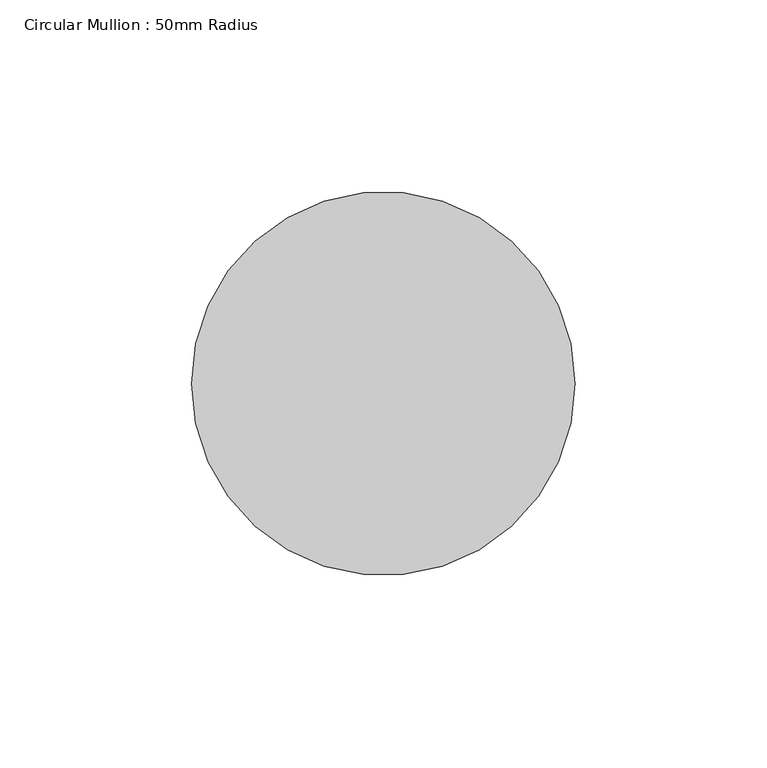
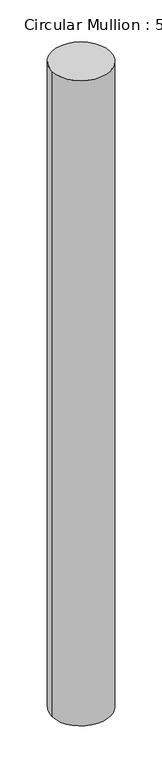
"""IFC4 building model written with IfcOpenShell, lengths in millimetres: member geometry, Circular Mullion : 50mm Radius."""

from ifc_helpers import new_model, si_unit, point, frame, origin, origin_2d, place, context, project, spatial, circle_curve, trimmed, segment, composite_curve, outline, extrude, source, transform, mapped, element, save


def circular_mullion_50mm_radius_3c5a0a30(model_context):
    return source(origin(), model_context, "Body", "SweptSolid", [
        extrude(outline(composite_curve([segment(trimmed(circle_curve(origin_2d(), 50.0), [point((50.0, 0.0))], [point((-50.0, 0.0))], False, "CARTESIAN"), True, "CONTINUOUS"), segment(trimmed(circle_curve(origin_2d(), 50.0), [point((-50.0, 0.0))], [point((50.0, 0.0))], False, "CARTESIAN"), True, "CONTINUOUS")], self_intersect=False)), frame((0.0, 0.0, -1167.7910831), z_axis=(0.0, 0.0, 1.0), x_axis=(1.0, 0.0, 0.0)), (0.0, 0.0, 1.0), 1167.7910831),
    ])


if __name__ == "__main__":
    model = new_model("IFC4")
    model_context = context("Model", 3, world=origin())
    ifc_project = project(units=[si_unit("LENGTHUNIT", "METRE", prefix="MILLI")], contexts=[model_context])
    site = spatial("IfcSite", under=ifc_project)
    building = spatial("IfcBuilding", under=site)
    placement = place(None, origin())
    circular_mullion_50mm_radius_shape = circular_mullion_50mm_radius_3c5a0a30(model_context)
    element("IfcMember", 1, ObjectType="Circular Mullion : 50mm Radius", at=placement, inside=building, context=model_context, shape_type="MappedRepresentation", body=[
        mapped(circular_mullion_50mm_radius_shape, transform((0.0, 0.0, 0.0), x_axis=(1.0, 0.0, 0.0), y_axis=(0.0, 1.0, 0.0), z_axis=(0.0, 0.0, 1.0))),
    ])
    save(model, "model.ifc")

# Revit data of these elements
# Type "Circular Mullion : 50mm Radius"
#   built-in parameter 1007350 = 0.164042 (stored number, unit not read)
# Element 1 (IfcMember, "Circular Mullion : 50mm Radius")
#   Materials on its faces: "Aluminium"
# Materials
#   "Aluminium": class "Metal", colour RGB 247 247 247, transparency 0, Description = "Aluminium 6061", Cost = 0
